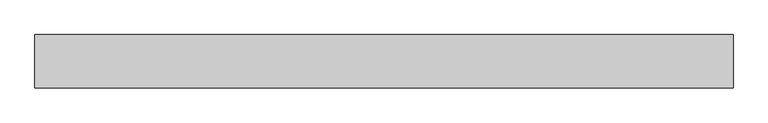
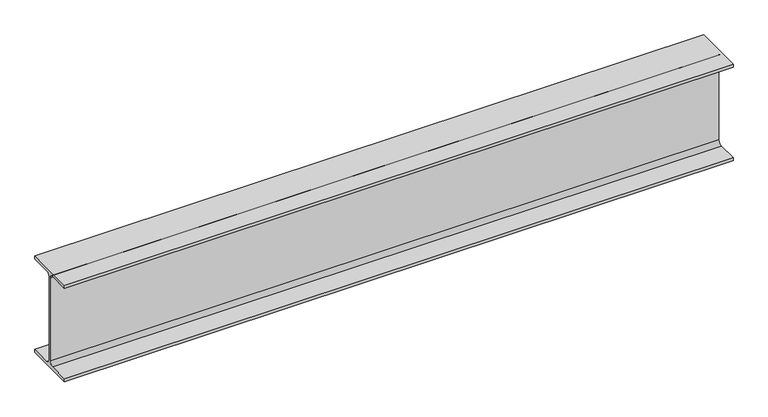
"""IFC4 building model written with IfcOpenShell, lengths in millimetres: beam geometry, 0912_Steel Framing_H-KSD3502 : H_SB_ASB_H-350x175x7x11."""

from ifc_helpers import new_model, si_unit, point, frame, frame_2d, origin, place, context, project, spatial, polyline, circle_curve, trimmed, segment, composite_curve, outline, extrude, source, transform, mapped, element, save


def beam_eb04396d(model_context):
    return source(origin(), model_context, "Body", "SweptSolid", [
        extrude(outline(composite_curve([segment(polyline([(87.5, -164.0), (87.5, -175.0), (-87.5, -175.0), (-87.5, -164.0), (-17.5, -164.0)]), True, "CONTINUOUS"), segment(trimmed(circle_curve(frame_2d((-17.5, -150.0)), 14.0), [point((-17.5, -164.0))], [point((-3.5, -150.0))], True, "CARTESIAN"), True, "CONTINUOUS"), segment(polyline([(-3.5, -150.0), (-3.5, 150.0)]), True, "CONTINUOUS"), segment(trimmed(circle_curve(frame_2d((-17.5, 150.0)), 14.0), [point((-3.5, 150.0))], [point((-17.5, 164.0))], True, "CARTESIAN"), True, "CONTINUOUS"), segment(polyline([(-17.5, 164.0), (-87.5, 164.0), (-87.5, 175.0), (87.5, 175.0), (87.5, 164.0), (17.5, 164.0)]), True, "CONTINUOUS"), segment(trimmed(circle_curve(frame_2d((17.5, 150.0)), 14.0), [point((17.5, 164.0))], [point((3.5, 150.0))], True, "CARTESIAN"), True, "CONTINUOUS"), segment(polyline([(3.5, 150.0), (3.5, -150.0)]), True, "CONTINUOUS"), segment(trimmed(circle_curve(frame_2d((17.5, -150.0)), 14.0), [point((3.5, -150.0))], [point((17.5, -164.0))], True, "CARTESIAN"), True, "CONTINUOUS"), segment(polyline([(17.5, -164.0), (87.5, -164.0)]), True, "CONTINUOUS")], self_intersect=False)), frame((-1146.3, 0.0, 0.0), z_axis=(1.0, 0.0, 0.0), x_axis=(0.0, 1.0, 0.0)), (0.0, 0.0, 1.0), 2292.6),
    ])


if __name__ == "__main__":
    model = new_model("IFC4")
    model_context = context("Model", 3, world=origin())
    ifc_project = project(units=[si_unit("LENGTHUNIT", "METRE", prefix="MILLI")], contexts=[model_context])
    site = spatial("IfcSite", under=ifc_project)
    building = spatial("IfcBuilding", under=site)
    placement = place(None, origin())
    beam_shape = beam_eb04396d(model_context)
    element("IfcBeam", 1, ObjectType="0912_Steel Framing_H-KSD3502 : H_SB_ASB_H-350x175x7x11", at=placement, inside=building, context=model_context, shape_type="MappedRepresentation", body=[
        mapped(beam_shape, transform((0.0, 0.0, 0.0), x_axis=(1.0, 0.0, 0.0), y_axis=(0.0, 1.0, 0.0), z_axis=(0.0, 0.0, 1.0))),
    ])
    save(model, "model.ifc")

# Revit data of these elements
# Type "0912_Steel Framing_H-KSD3502 : H_SB_ASB_H-350x175x7x11"
#   H_WM Code_1 = "S01AA002-00001 | Main Steel Structure Fabrication Work | Shelter/Building | Medium Steel - Standard (90KG/M>Weight≥30KG/M) | Material: (   )"
#   H_WM Code_2 = "S03AA028-00001 | Main Steel Structure Erection Work | Shelter/Building | Medium Steel (90KG/M>Weight≥30KG/M) | Material: (   )"
#   H_WM Code_3 = "S01AA010-00001 | Main Steel Structure Fabrication Work | Shelter/Building | Steel Painting/Coating | for Non-Fireproofed Steel Surface, Surface Preparation, Primer, Second & Final Coat | Material: (   )"
#   H_Q'ty Cal Type Tag = "SB-Q2"
#   Width = 17.5 cm
#   Web Thickness = 0.7 cm
#   Web Fillet = 1.4 cm
#   Warping Constant = 282000.0 cm⁶
#   W = 0
#   Torsional Moment of Inertia = 19.4042 cm⁴
#   Section Area = 63.14 cm²
#   Plastic Modulus weak axis = 174.0 cm³
#   Plastic Modulus strong axis = 868.0 cm³
#   Perimeter = 1.36 m²/m
#   Nominal Weight = 49.60 kgf/m
#   Moment of Inertia weak axis = 984.00 cm⁴
#   Moment of Inertia strong axis = 13600.00 cm⁴
#   Height = 35.0 cm
#   Flange Thickness = 1.1 cm
#   Elastic Modulus weak axis = 112.0 cm³
#   Elastic Modulus strong axis = 775.0 cm³
#   Centroid Vertical = 17.5 cm
#   Centroid Horizontal = 8.75 cm
#   Ix = 136000000
#   Length [instance default] = 1.5240 m
#   Zx = 868000
#   b = 0.1750 m
#   h = 0.3500 m
#   r = 0.0140 m
#   s = 0.0070 m
#   t = 0.0110 m
#   A = 0.006314 m²
#   Structural Material [instance default] = Steel, 45-345
#   Assembly Code = ""
# Element 1 (IfcBeam, "0912_Steel Framing_H-KSD3502 : H_SB_ASB_H-350x175x7x11")
#   Structural Material = none
# Materials
#   "Steel, 45-345": class "Metal", colour RGB 189 187 185, transparency 0, Description = "Steel 345 MPa", Cost = 0
